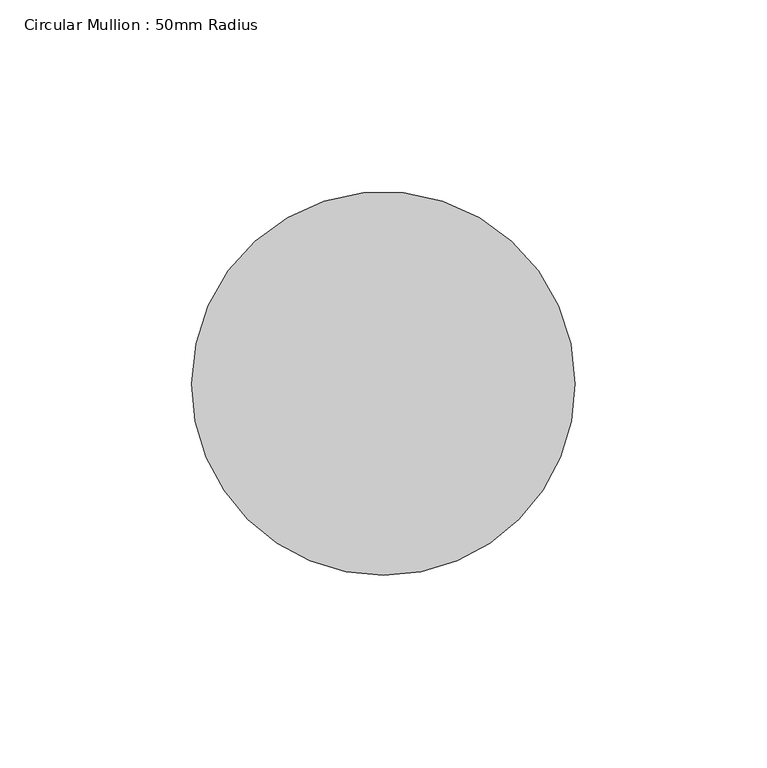
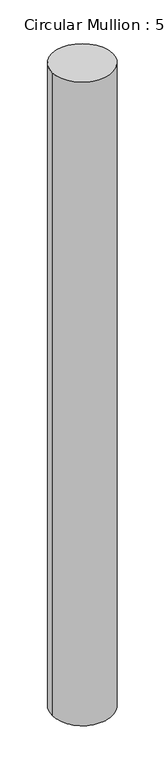
"""IFC4 building model written with IfcOpenShell, lengths in millimetres: member geometry, Circular Mullion : 50mm Radius."""

from ifc_helpers import new_model, si_unit, frame, origin, place, context, project, spatial, ellipse_curve, source, transform, mapped, element, save
from ifc_brep_helpers import plane_surface, cylinder_surface, advanced_brep


def circular_mullion_50mm_radius_b3aecd9d(model_context):
    return source(origin(), model_context, "Body", "AdvancedBrep", [
        advanced_brep(
        [(-100.0, 0.0, 1.2148663), (0.0, 0.0, 0.0), (0.0, 0.0, -1122.8231585), (-100.0, 0.0, -1124.1048355)],
        [
            (0, 1, ellipse_curve(frame((-50.0, 0.0, 0.6074332), z_axis=(-0.012145168294368793, -0.02068286419235582, -0.9997123156268017), x_axis=(-0.5062169499640441, -0.8620725686303924, 0.023985120055941472)), 50.0143884, 50.0)),
            (1, 2),
            (2, 3, ellipse_curve(frame((-50.0, 0.0, -1123.463997), z_axis=(-0.012812666617103785, -0.021819594192561603, 0.999679819183838), x_axis=(0.5062004949799549, 0.8620445462767453, 0.025303342003953042)), 50.0160142, 50.0)),
            (3, 0),
            (1, 0, ellipse_curve(frame((-50.0, 0.0, 0.6074332), z_axis=(-0.012145168294368793, -0.02068286419235582, -0.9997123156268017), x_axis=(-0.5062169499640441, -0.8620725686303924, 0.023985120055941472)), 50.0143884, 50.0)),
            (3, 2, ellipse_curve(frame((-50.0, 0.0, -1123.463997), z_axis=(-0.012812666617103785, -0.021819594192561603, 0.999679819183838), x_axis=(0.5062004949799549, 0.8620445462767453, 0.025303342003953042)), 50.0160142, 50.0)),
        ],
        [
            cylinder_surface(frame((-50.0, 0.0, 0.0), z_axis=(0.0, 0.0, 1.0), x_axis=(1.0, 0.0, 0.0)), 50.0),
            plane_surface(frame((-262.8353325, 154.3393274, 0.0), z_axis=(0.012145168294368793, 0.02068286419235582, 0.9997123156268017), x_axis=(0.5062169499640461, 0.8620725686303913, -0.02398512005594251))),
            plane_surface(frame((-262.8353325, 154.3393274, -1122.8231585), z_axis=(0.012812666617103789, 0.021819594192561607, -0.9996798191838382), x_axis=(0.506200494979955, 0.8620445462767453, 0.02530334200395501))),
        ],
        [
            (0, [[1, 2, 3, 4]]),
            (0, [[5, -4, 6, -2]]),
            (1, [[-1, -5]]),
            (2, [[-6, -3]]),
        ],
    ),
    ])


if __name__ == "__main__":
    model = new_model("IFC4")
    model_context = context("Model", 3, world=origin())
    ifc_project = project(units=[si_unit("LENGTHUNIT", "METRE", prefix="MILLI")], contexts=[model_context])
    site = spatial("IfcSite", under=ifc_project)
    building = spatial("IfcBuilding", under=site)
    placement = place(None, origin())
    circular_mullion_50mm_radius_shape = circular_mullion_50mm_radius_b3aecd9d(model_context)
    element("IfcMember", 1, ObjectType="Circular Mullion : 50mm Radius", at=placement, inside=building, context=model_context, shape_type="MappedRepresentation", body=[
        mapped(circular_mullion_50mm_radius_shape, transform((0.0, 0.0, 0.0), x_axis=(1.0, 0.0, 0.0), y_axis=(0.0, 1.0, 0.0), z_axis=(0.0, 0.0, 1.0))),
    ])
    save(model, "model.ifc")

# Revit data of these elements
# Type "Circular Mullion : 50mm Radius"
#   built-in parameter 1007350 = 0.164042 (stored number, unit not read)
# Element 1 (IfcMember, "Circular Mullion : 50mm Radius")
#   Materials on its faces: "Aluminium"
# Materials
#   "Aluminium": class "Metal", colour RGB 247 247 247, transparency 0, Description = "Aluminium 6061", Cost = 0
